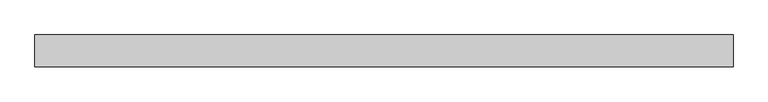
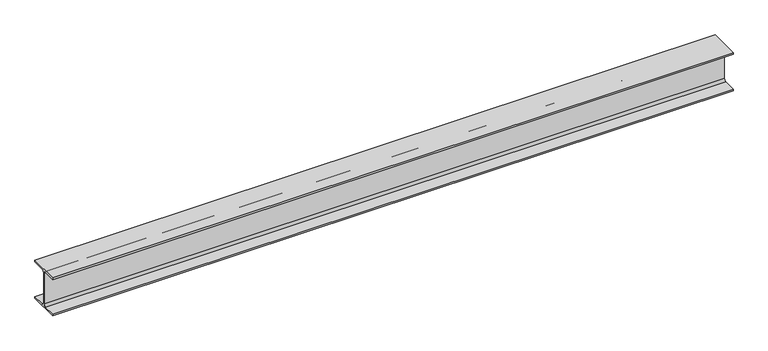
"""IFC4 building model written with IfcOpenShell, lengths in millimetres: beam geometry, 0912_Steel Framing_H-KSD3502 : H_SB_ASB_H-390x300x10x16."""

from ifc_helpers import new_model, si_unit, point, frame, frame_2d, origin, place, context, project, spatial, polyline, circle_curve, trimmed, segment, composite_curve, outline, extrude, source, transform, mapped, element, save


def beam_f1fc430e(model_context):
    return source(origin(), model_context, "Body", "SweptSolid", [
        extrude(outline(composite_curve([segment(polyline([(150.0, -179.0), (150.0, -195.0), (-150.0, -195.0), (-150.0, -179.0), (-27.0, -179.0)]), True, "CONTINUOUS"), segment(trimmed(circle_curve(frame_2d((-27.0, -157.0)), 22.0), [point((-27.0, -179.0))], [point((-5.0, -157.0))], True, "CARTESIAN"), True, "CONTINUOUS"), segment(polyline([(-5.0, -157.0), (-5.0, 157.0)]), True, "CONTINUOUS"), segment(trimmed(circle_curve(frame_2d((-27.0, 157.0)), 22.0), [point((-5.0, 157.0))], [point((-27.0, 179.0))], True, "CARTESIAN"), True, "CONTINUOUS"), segment(polyline([(-27.0, 179.0), (-150.0, 179.0), (-150.0, 195.0), (150.0, 195.0), (150.0, 179.0), (27.0, 179.0)]), True, "CONTINUOUS"), segment(trimmed(circle_curve(frame_2d((27.0, 157.0)), 22.0), [point((27.0, 179.0))], [point((5.0, 157.0))], True, "CARTESIAN"), True, "CONTINUOUS"), segment(polyline([(5.0, 157.0), (5.0, -157.0)]), True, "CONTINUOUS"), segment(trimmed(circle_curve(frame_2d((27.0, -157.0)), 22.0), [point((5.0, -157.0))], [point((27.0, -179.0))], True, "CARTESIAN"), True, "CONTINUOUS"), segment(polyline([(27.0, -179.0), (150.0, -179.0)]), True, "CONTINUOUS")], self_intersect=False)), frame((-3262.3, 0.0, 0.0), z_axis=(1.0, 0.0, 0.0), x_axis=(0.0, 1.0, 0.0)), (0.0, 0.0, 1.0), 6599.6),
    ])


if __name__ == "__main__":
    model = new_model("IFC4")
    model_context = context("Model", 3, world=origin())
    ifc_project = project(units=[si_unit("LENGTHUNIT", "METRE", prefix="MILLI")], contexts=[model_context])
    site = spatial("IfcSite", under=ifc_project)
    building = spatial("IfcBuilding", under=site)
    placement = place(None, origin())
    beam_shape = beam_f1fc430e(model_context)
    element("IfcBeam", 1, ObjectType="0912_Steel Framing_H-KSD3502 : H_SB_ASB_H-390x300x10x16", at=placement, inside=building, context=model_context, shape_type="MappedRepresentation", body=[
        mapped(beam_shape, transform((0.0, 0.0, 0.0), x_axis=(1.0, 0.0, 0.0), y_axis=(0.0, 1.0, 0.0), z_axis=(0.0, 0.0, 1.0))),
    ])
    save(model, "model.ifc")

# Revit data of these elements
# Type "0912_Steel Framing_H-KSD3502 : H_SB_ASB_H-390x300x10x16"
#   H_WM Code_1 = "S01AA001-00001 | Main Steel Structure Fabrication Work | Shelter/Building | Heavy Steel - Standard (Weight≥90KG/M) | Material: (   )"
#   H_WM Code_2 = "S03AA027-00001 | Main Steel Structure Erection Work | Shelter/Building | Heavy Steel (Weight≥90KG/M) | Material: (   )"
#   H_WM Code_3 = "S01AA010-00001 | Main Steel Structure Fabrication Work | Shelter/Building | Steel Painting/Coating | for Non-Fireproofed Steel Surface, Surface Preparation, Primer, Second & Final Coat | Material: (   )"
#   H_Q'ty Cal Type Tag = "SB-Q2"
#   Width = 30.0 cm
#   Web Thickness = 1.0 cm
#   Web Fillet = 2.2 cm
#   Warping Constant = 2520000.0 cm⁶
#   W = 0
#   Torsional Moment of Inertia = 94.3867 cm⁴
#   Section Area = 136.0 cm²
#   Plastic Modulus weak axis = 733.0 cm³
#   Plastic Modulus strong axis = 2190.0 cm³
#   Perimeter = 1.92 m²/m
#   Nominal Weight = 107.00 kgf/m
#   Moment of Inertia weak axis = 7210.00 cm⁴
#   Moment of Inertia strong axis = 38700.00 cm⁴
#   Height = 39.0 cm
#   Flange Thickness = 1.6 cm
#   Elastic Modulus weak axis = 481.0 cm³
#   Elastic Modulus strong axis = 1980.0 cm³
#   Centroid Vertical = 19.5 cm
#   Centroid Horizontal = 15.0 cm
#   Ix = 387000000
#   Length [instance default] = 1.5240 m
#   Zx = 2190000
#   b = 0.3000 m
#   h = 0.3900 m
#   r = 0.0220 m
#   s = 0.0100 m
#   t = 0.0160 m
#   A = 0.0136 m²
#   Structural Material [instance default] = Steel, 45-345
#   Assembly Code = ""
# Element 1 (IfcBeam, "0912_Steel Framing_H-KSD3502 : H_SB_ASB_H-390x300x10x16")
#   Structural Material = none
# Materials
#   "Steel, 45-345": class "Metal", colour RGB 189 187 185, transparency 0, Description = "Steel 345 MPa", Cost = 0
